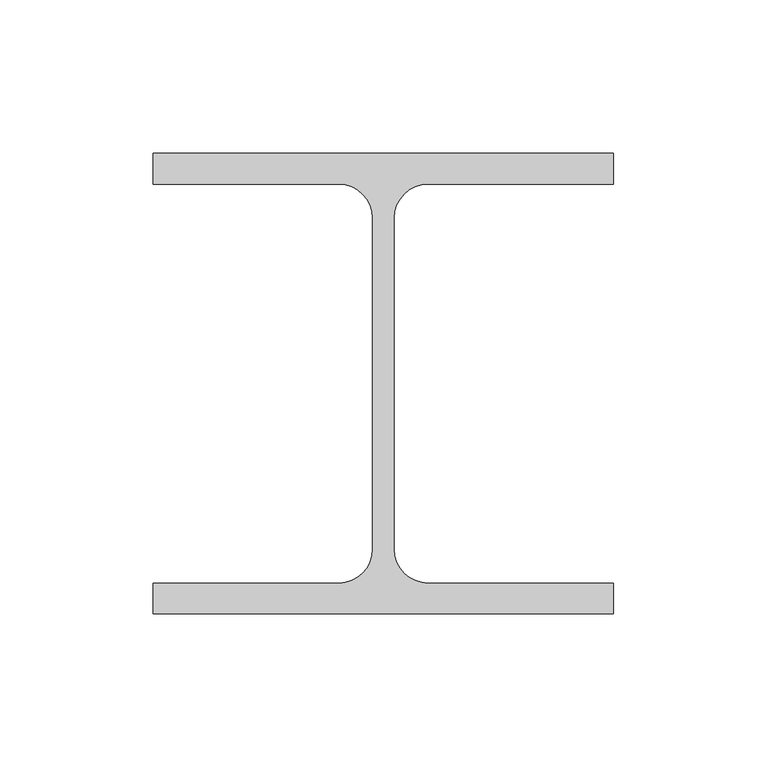
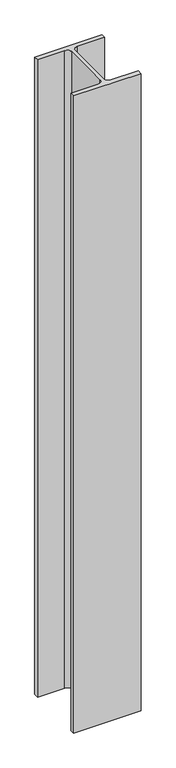
"""IFC4 building model written with IfcOpenShell, lengths in millimetres: column geometry, 0912_Steel Column_H_KSD3502 : H_SC_ASC_H-150x150x7x10."""

from ifc_helpers import new_model, si_unit, point, frame, frame_2d, origin, place, context, project, spatial, polyline, circle_curve, trimmed, segment, composite_curve, outline, extrude, source, transform, mapped, element, save


def column_24869f1c(model_context):
    return source(origin(), model_context, "Body", "SweptSolid", [
        extrude(outline(composite_curve([segment(polyline([(75.0, 75.0), (75.0, 65.0), (14.5, 65.0)]), True, "CONTINUOUS"), segment(trimmed(circle_curve(frame_2d((14.5, 54.0)), 11.0), [point((14.5, 65.0))], [point((3.5, 54.0))], True, "CARTESIAN"), True, "CONTINUOUS"), segment(polyline([(3.5, 54.0), (3.5, -54.0)]), True, "CONTINUOUS"), segment(trimmed(circle_curve(frame_2d((14.5, -54.0)), 11.0), [point((3.5, -54.0))], [point((14.5, -65.0))], True, "CARTESIAN"), True, "CONTINUOUS"), segment(polyline([(14.5, -65.0), (75.0, -65.0), (75.0, -75.0), (-75.0, -75.0), (-75.0, -65.0), (-14.5, -65.0)]), True, "CONTINUOUS"), segment(trimmed(circle_curve(frame_2d((-14.5, -54.0)), 11.0), [point((-14.5, -65.0))], [point((-3.5, -54.0))], True, "CARTESIAN"), True, "CONTINUOUS"), segment(polyline([(-3.5, -54.0), (-3.5, 54.0)]), True, "CONTINUOUS"), segment(trimmed(circle_curve(frame_2d((-14.5, 54.0)), 11.0), [point((-3.5, 54.0))], [point((-14.5, 65.0))], True, "CARTESIAN"), True, "CONTINUOUS"), segment(polyline([(-14.5, 65.0), (-75.0, 65.0), (-75.0, 75.0), (75.0, 75.0)]), True, "CONTINUOUS")], self_intersect=False)), frame((0.0, 0.0, 17299.9720055), z_axis=(0.0, 0.0, 1.0), x_axis=(1.0, 0.0, 0.0)), (0.0, 0.0, 1.0), 1500.0),
    ])


if __name__ == "__main__":
    model = new_model("IFC4")
    model_context = context("Model", 3, world=origin())
    ifc_project = project(units=[si_unit("LENGTHUNIT", "METRE", prefix="MILLI")], contexts=[model_context])
    site = spatial("IfcSite", under=ifc_project)
    building = spatial("IfcBuilding", under=site)
    placement = place(None, origin())
    column_shape = column_24869f1c(model_context)
    element("IfcColumn", 1, ObjectType="0912_Steel Column_H_KSD3502 : H_SC_ASC_H-150x150x7x10", at=placement, inside=building, context=model_context, shape_type="MappedRepresentation", body=[
        mapped(column_shape, transform((0.0, 0.0, 0.0), x_axis=(1.0, 0.0, 0.0), y_axis=(0.0, 1.0, 0.0), z_axis=(0.0, 0.0, 1.0))),
    ])
    save(model, "model.ifc")

# Revit data of these elements
# Type "0912_Steel Column_H_KSD3502 : H_SC_ASC_H-150x150x7x10"
#   H_WM Code_1 = "S01AA002-00001 | Main Steel Structure Fabrication Work | Shelter/Building | Medium Steel - Standard (90KG/M>Weight≥30KG/M) | Material: (   )"
#   H_WM Code_2 = "S03AA028-00001 | Main Steel Structure Erection Work | Shelter/Building | Medium Steel (90KG/M>Weight≥30KG/M) | Material: (   )"
#   H_WM Code_3 = "S01AA010-00001 | Main Steel Structure Fabrication Work | Shelter/Building | Steel Painting/Coating | for Non-Fireproofed Steel Surface, Surface Preparation, Primer, Second & Final Coat | Material: (   )"
#   H_Q'ty Cal Type Tag = "SC-Q2"
#   Width = 15.0 cm
#   Web Thickness = 0.7 cm
#   Web Fillet = 1.1 cm
#   Warping Constant = 27562.5 cm⁶
#   Torsional Moment of Inertia = 11.6007 cm⁴
#   Section Area = 40.14 cm²
#   Plastic Modulus weak axis = 115.0 cm³
#   Plastic Modulus strong axis = 246.0 cm³
#   Perimeter = 0.87 m²/m
#   Nominal Weight = 31.50 kgf/m
#   Moment of Inertia weak axis = 563.00 cm⁴
#   Moment of Inertia strong axis = 1640.00 cm⁴
#   Height = 15.0 cm
#   Flange Thickness = 1.0 cm
#   Elastic Modulus weak axis = 75.1 cm³
#   Elastic Modulus strong axis = 219.0 cm³
#   Centroid Vertical = 7.5 cm
#   Centroid Horizontal = 7.5 cm
#   Structural Material [instance default] = Steel, 45-345
#   Section Name Key = ""
#   Bolt Spacing = 0
#   Assembly Code = ""
# Element 1 (IfcColumn, "0912_Steel Column_H_KSD3502 : H_SC_ASC_H-150x150x7x10")
#   Structural Material = none
# Materials
#   "Steel, 45-345": class "Metal", colour RGB 189 187 185, transparency 0, Description = "Steel 345 MPa", Cost = 0
